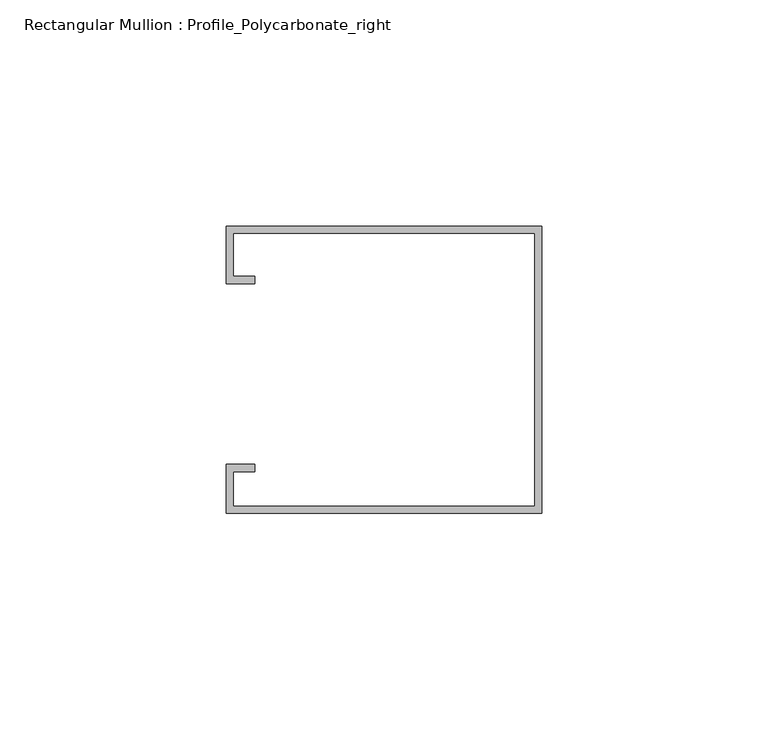
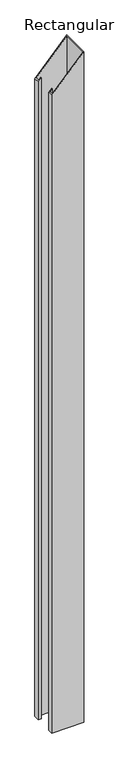
"""IFC4 building model written with IfcOpenShell, lengths in millimetres: member geometry, Rectangular Mullion : Profile_Polycarbonate_right."""

from ifc_helpers import new_model, si_unit, origin, place, context, project, spatial, faceted_brep, source, transform, mapped, element, save


def rectangular_mullion_profile_polycarbonate_right_fcf1ccf7(model_context):
    return source(origin(), model_context, "Body", "Brep", [
        faceted_brep([(0.0, 32.7, -1543.7114583), (0.0, -30.8, -1543.7114583), (-69.85, -30.8, -1543.7114583), (-69.85, -20.0, -1543.7114583), (-63.5, -20.0, -1543.7114583), (-63.5, -21.5875, -1543.7114583), (-68.2625, -21.5875, -1543.7114583), (-68.2625, -29.2125, -1543.7114583), (-1.5875, -29.2125, -1543.7114583), (-1.5875, 31.1125, -1543.7114583), (-68.2625, 31.1125, -1543.7114583), (-68.2625, 21.5875, -1543.7114583), (-63.5, 21.5875, -1543.7114583), (-63.5, 20.0, -1543.7114583), (-69.85, 20.0, -1543.7114583), (-69.85, 32.7, -1543.7114583), (-69.85, 32.7, -75.9129484), (0.0, 32.7, 0.0), (-69.85, 20.0, -75.9129484), (-63.5, 20.0, -69.0117713), (-63.5, 21.5875, -69.0117713), (-68.2625, 21.5875, -74.1876542), (-68.2625, 31.1125, -74.1876542), (-1.5875, 31.1125, -1.7252943), (-1.5875, -29.2125, -1.7252943), (-68.2625, -29.2125, -74.1876542), (-68.2625, -21.5875, -74.1876542), (-63.5, -21.5875, -69.0117713), (-63.5, -20.0, -69.0117713), (-69.85, -20.0, -75.9129484), (-69.85, -30.8, -75.9129484), (0.0, -30.8, 0.0)], [[[0, 1, 2, 3, 4, 5, 6, 7, 8, 9, 10, 11, 12, 13, 14, 15]], [[16, 17, 0, 15]], [[18, 16, 15, 14]], [[19, 18, 14, 13]], [[20, 19, 13, 12]], [[21, 20, 12, 11]], [[22, 21, 11, 10]], [[23, 22, 10, 9]], [[24, 23, 9, 8]], [[25, 24, 8, 7]], [[26, 25, 7, 6]], [[27, 26, 6, 5]], [[28, 27, 5, 4]], [[29, 28, 4, 3]], [[30, 29, 3, 2]], [[31, 30, 2, 1]], [[17, 31, 1, 0]], [[17, 16, 18, 19, 20, 21, 22, 23, 24, 25, 26, 27, 28, 29, 30, 31]]]),
    ])


if __name__ == "__main__":
    model = new_model("IFC4")
    model_context = context("Model", 3, world=origin())
    ifc_project = project(units=[si_unit("LENGTHUNIT", "METRE", prefix="MILLI")], contexts=[model_context])
    site = spatial("IfcSite", under=ifc_project)
    building = spatial("IfcBuilding", under=site)
    placement = place(None, origin())
    rectangular_mullion_profile_polycarbonate_right_shape = rectangular_mullion_profile_polycarbonate_right_fcf1ccf7(model_context)
    element("IfcMember", 1, ObjectType="Rectangular Mullion : Profile_Polycarbonate_right", at=placement, inside=building, context=model_context, shape_type="MappedRepresentation", body=[
        mapped(rectangular_mullion_profile_polycarbonate_right_shape, transform((0.0, 0.0, 0.0), x_axis=(1.0, 0.0, 0.0), y_axis=(0.0, 1.0, 0.0), z_axis=(0.0, 0.0, 1.0))),
    ])
    save(model, "model.ifc")

# Revit data of these elements
# Type "Rectangular Mullion : Profile_Polycarbonate_right"
#   built-in parameter 1007322 = 0.208333 (stored number, unit not read)
#   built-in parameter 1007321 = 0 (stored number, unit not read)
#   built-in parameter 1007320 = 0.00520833 (stored number, unit not read)
# Element 1 (IfcMember, "Rectangular Mullion : Profile_Polycarbonate_right")
#   Materials on its faces: "ALUMINUM PROFILE AT POLYCARBONATE PANEL"
# Materials
#   "ALUMINUM PROFILE AT POLYCARBONATE PANEL": class "Metal", colour RGB 244 244 244, transparency 0, Description = "Aluminum 6061", Cost = 0
